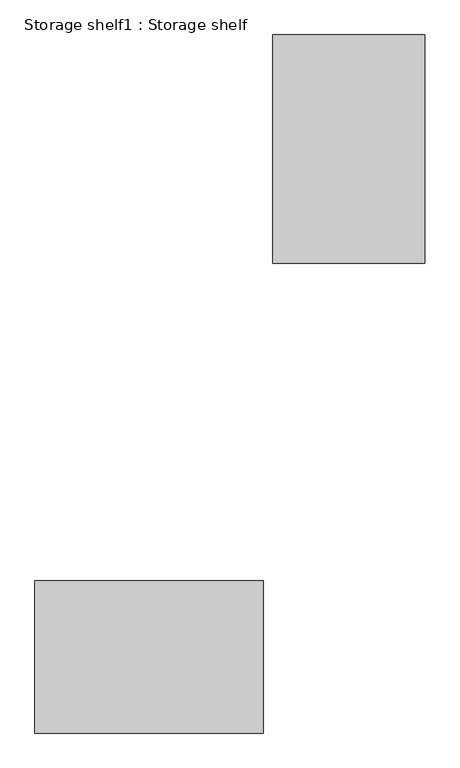
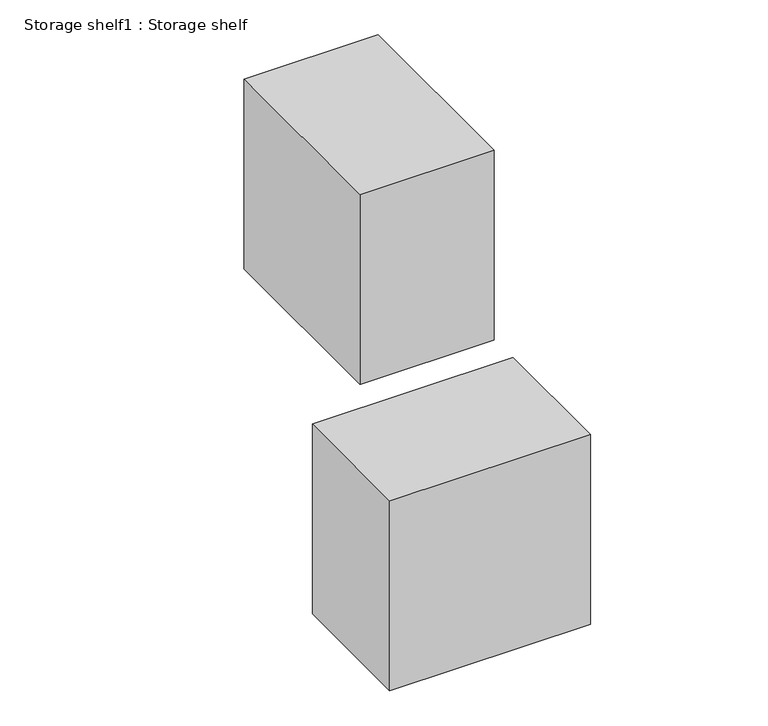
"""IFC4 building model written with IfcOpenShell, lengths in millimetres: furniture geometry, Storage shelf1 : Storage shelf."""

from ifc_helpers import new_model, si_unit, origin, origin_with_axes, place, context, project, spatial, polyline, outline, extrude, source, transform, mapped, element, save


def storage_shelf1_storage_shelf_d4849a82(model_context):
    return source(origin(), model_context, "Body", "SweptSolid", [
        extrude(outline(polyline([(28842.4870052, 7913.3615366), (28232.8870052, 7913.3615366), (28232.8870052, 8827.7615366), (28842.4870052, 8827.7615366), (28842.4870052, 7913.3615366)])), origin_with_axes(), (0.0, 0.0, 1.0), 914.4),
        extrude(outline(polyline([(28195.0605411, 6639.4562521), (28195.0605411, 6029.8562521), (27280.6605411, 6029.8562521), (27280.6605411, 6639.4562521), (28195.0605411, 6639.4562521)])), origin_with_axes(), (0.0, 0.0, 1.0), 914.4),
    ])


if __name__ == "__main__":
    model = new_model("IFC4")
    model_context = context("Model", 3, world=origin())
    ifc_project = project(units=[si_unit("LENGTHUNIT", "METRE", prefix="MILLI")], contexts=[model_context])
    site = spatial("IfcSite", under=ifc_project)
    building = spatial("IfcBuilding", under=site)
    placement = place(None, origin())
    storage_shelf1_storage_shelf_shape = storage_shelf1_storage_shelf_d4849a82(model_context)
    element("IfcFurniture", 1, ObjectType="Storage shelf1 : Storage shelf", at=placement, inside=building, context=model_context, shape_type="MappedRepresentation", body=[
        mapped(storage_shelf1_storage_shelf_shape, transform((0.0, 0.0, 0.0), x_axis=(1.0, 0.0, 0.0), y_axis=(0.0, 1.0, 0.0), z_axis=(0.0, 0.0, 1.0))),
    ])
    save(model, "model.ifc")
